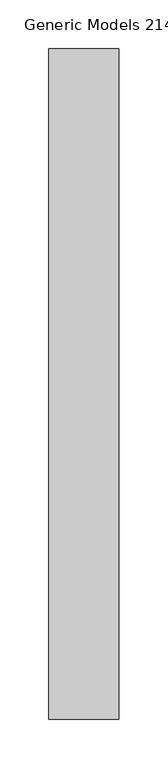
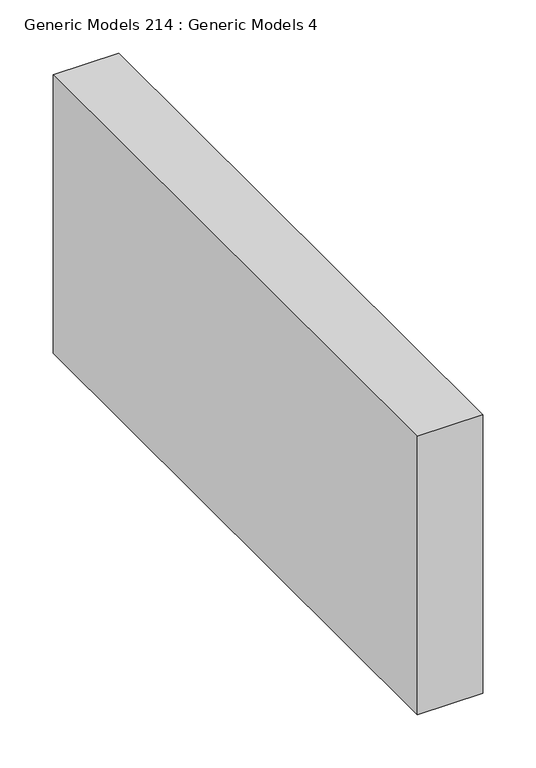
"""IFC4 building model written with IfcOpenShell, lengths in millimetres: proxy geometry, Generic Models 214 : Generic Models 4."""

from ifc_helpers import new_model, si_unit, frame, origin, place, context, project, spatial, polyline, outline, extrude, source, transform, mapped, element, save


def generic_models_214_generic_models_4_f71f5e20(model_context):
    return source(origin(), model_context, "Body", "SweptSolid", [
        extrude(outline(polyline([(-318.6717702, 1085.2769662), (-247.1350514, 1085.2769662), (-247.1350514, 399.7309662), (-318.6717702, 399.7309662), (-318.6717702, 1085.2769662)])), frame((0.0, 0.0, 126340.2389687), z_axis=(0.0, 0.0, 1.0), x_axis=(1.0, 0.0, 0.0)), (0.0, 0.0, 1.0), 320.0796875),
    ])


if __name__ == "__main__":
    model = new_model("IFC4")
    model_context = context("Model", 3, world=origin())
    ifc_project = project(units=[si_unit("LENGTHUNIT", "METRE", prefix="MILLI")], contexts=[model_context])
    site = spatial("IfcSite", under=ifc_project)
    building = spatial("IfcBuilding", under=site)
    placement = place(None, origin())
    generic_models_214_generic_models_4_shape = generic_models_214_generic_models_4_f71f5e20(model_context)
    element("IfcBuildingElementProxy", 1, Name="Generic Models 214 : Generic Models 4", ObjectType="Generic Models 214 : Generic Models 4", at=placement, inside=building, context=model_context, shape_type="MappedRepresentation", body=[
        mapped(generic_models_214_generic_models_4_shape, transform((0.0, 0.0, 0.0), x_axis=(1.0, 0.0, 0.0), y_axis=(0.0, 1.0, 0.0), z_axis=(0.0, 0.0, 1.0))),
    ])
    save(model, "model.ifc")

# Revit data of these elements
# Element 1 (IfcBuildingElementProxy, "Generic Models 214 : Generic Models 4")
#   Materials on its faces: "_BLOCKING AS REQUIRED"
# Materials
#   "_BLOCKING AS REQUIRED": class "Generic", colour RGB 177 130 114, transparency 0, Cost = 0
